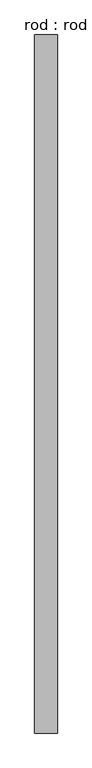
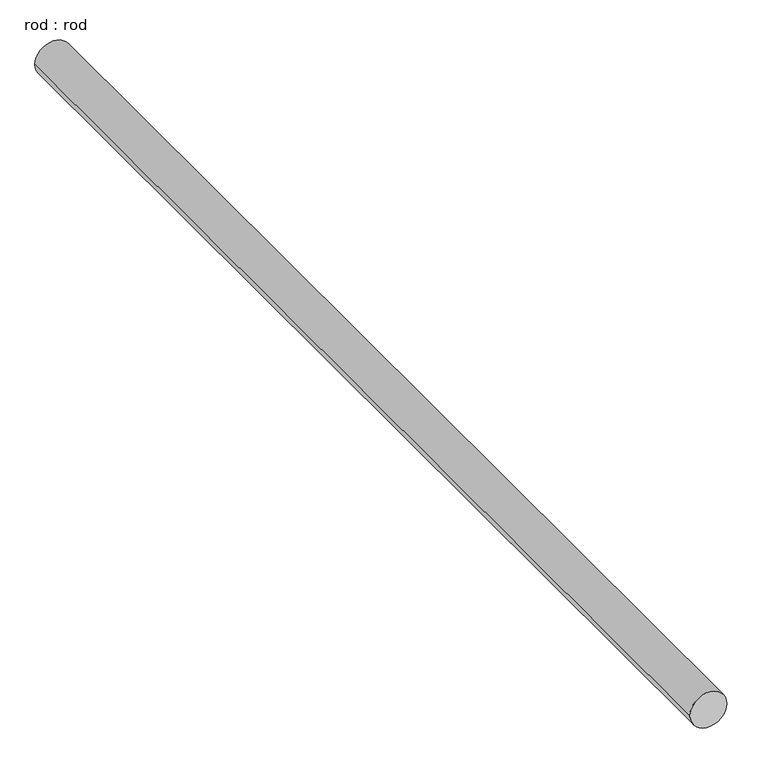
"""IFC4 building model written with IfcOpenShell, lengths in millimetres: proxy geometry, rod : rod."""

from ifc_helpers import new_model, si_unit, point, frame, frame_2d, origin, place, context, project, spatial, circle_curve, trimmed, segment, composite_curve, outline, extrude, source, transform, mapped, element, save


def rod_rod_0cc72d16(model_context):
    return source(origin(), model_context, "Body", "SweptSolid", [
        extrude(outline(composite_curve([segment(trimmed(circle_curve(frame_2d((0.0108462, 0.0)), 200.0), [point((0.0108462, 200.0))], [point((0.0108462, -200.0))], False, "CARTESIAN"), True, "CONTINUOUS"), segment(trimmed(circle_curve(frame_2d((0.0108462, 0.0)), 200.0), [point((0.0108462, -200.0))], [point((0.0108462, 200.0))], False, "CARTESIAN"), True, "CONTINUOUS")], self_intersect=False)), frame((0.0, -2085.8428132, 0.0), z_axis=(0.0, 1.0, 0.0), x_axis=(0.0, 0.0, 1.0)), (0.0, 0.0, 1.0), 12357.1428571),
    ])


if __name__ == "__main__":
    model = new_model("IFC4")
    model_context = context("Model", 3, world=origin())
    ifc_project = project(units=[si_unit("LENGTHUNIT", "METRE", prefix="MILLI")], contexts=[model_context])
    site = spatial("IfcSite", under=ifc_project)
    building = spatial("IfcBuilding", under=site)
    placement = place(None, origin())
    rod_rod_shape = rod_rod_0cc72d16(model_context)
    element("IfcBuildingElementProxy", 1, Name="rod : rod", ObjectType="rod : rod", at=placement, inside=building, context=model_context, shape_type="MappedRepresentation", body=[
        mapped(rod_rod_shape, transform((0.0, 0.0, 0.0), x_axis=(1.0, 0.0, 0.0), y_axis=(0.0, 1.0, 0.0), z_axis=(0.0, 0.0, 1.0))),
    ])
    save(model, "model.ifc")

# Revit data of these elements
# Type "rod : rod"
#   Default Elevation = 0
